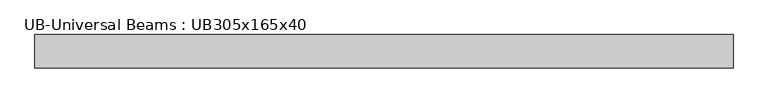
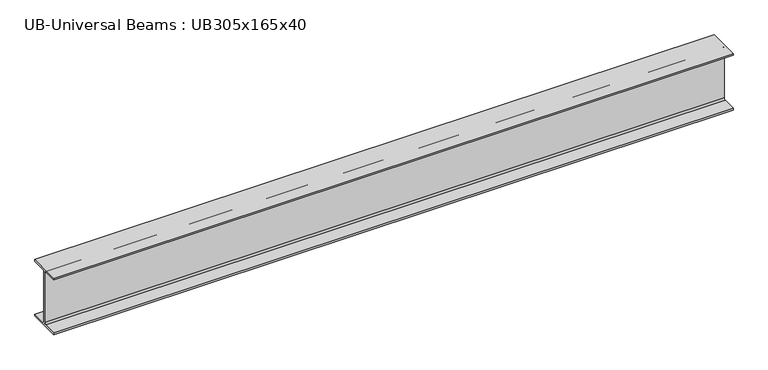
"""IFC4 building model written with IfcOpenShell, lengths in millimetres: beam geometry, UB-Universal Beams : UB305x165x40."""

from ifc_helpers import new_model, si_unit, point, frame, frame_2d, origin, place, context, project, spatial, polyline, circle_curve, trimmed, segment, composite_curve, outline, extrude, source, transform, mapped, element, save


def ub_universal_beams_ub305x165x40_daa15f39(model_context):
    return source(origin(), model_context, "Body", "SweptSolid", [
        extrude(outline(composite_curve([segment(polyline([(82.5, -141.5), (82.5, -151.7), (-82.5, -151.7), (-82.5, -141.5), (-11.9, -141.5)]), True, "CONTINUOUS"), segment(trimmed(circle_curve(frame_2d((-11.9, -132.6)), 8.9), [point((-11.9, -141.5))], [point((-3.0, -132.6))], True, "CARTESIAN"), True, "CONTINUOUS"), segment(polyline([(-3.0, -132.6), (-3.0, 132.6)]), True, "CONTINUOUS"), segment(trimmed(circle_curve(frame_2d((-11.9, 132.6)), 8.9), [point((-3.0, 132.6))], [point((-11.9, 141.5))], True, "CARTESIAN"), True, "CONTINUOUS"), segment(polyline([(-11.9, 141.5), (-82.5, 141.5), (-82.5, 151.7), (82.5, 151.7), (82.5, 141.5), (11.9, 141.5)]), True, "CONTINUOUS"), segment(trimmed(circle_curve(frame_2d((11.9, 132.6)), 8.9), [point((11.9, 141.5))], [point((3.0, 132.6))], True, "CARTESIAN"), True, "CONTINUOUS"), segment(polyline([(3.0, 132.6), (3.0, -132.6)]), True, "CONTINUOUS"), segment(trimmed(circle_curve(frame_2d((11.9, -132.6)), 8.9), [point((3.0, -132.6))], [point((11.9, -141.5))], True, "CARTESIAN"), True, "CONTINUOUS"), segment(polyline([(11.9, -141.5), (82.5, -141.5)]), True, "CONTINUOUS")], self_intersect=False)), frame((-1724.05, 0.0, 0.0), z_axis=(1.0, 0.0, 0.0), x_axis=(0.0, 1.0, 0.0)), (0.0, 0.0, 1.0), 3448.1),
    ])


if __name__ == "__main__":
    model = new_model("IFC4")
    model_context = context("Model", 3, world=origin())
    ifc_project = project(units=[si_unit("LENGTHUNIT", "METRE", prefix="MILLI")], contexts=[model_context])
    site = spatial("IfcSite", under=ifc_project)
    building = spatial("IfcBuilding", under=site)
    placement = place(None, origin())
    ub_universal_beams_ub305x165x40_shape = ub_universal_beams_ub305x165x40_daa15f39(model_context)
    element("IfcBeam", 1, ObjectType="UB-Universal Beams : UB305x165x40", at=placement, inside=building, context=model_context, shape_type="MappedRepresentation", body=[
        mapped(ub_universal_beams_ub305x165x40_shape, transform((0.0, 0.0, 0.0), x_axis=(1.0, 0.0, 0.0), y_axis=(0.0, 1.0, 0.0), z_axis=(0.0, 0.0, 1.0))),
    ])
    save(model, "model.ifc")

# Revit data of these elements
# Type "UB-Universal Beams : UB305x165x40"
#   Section Name Key = "UB305X165X40"
#   Width = 16.5 cm
#   Web Thickness = 0.6 cm
#   Web Fillet = 0.89 cm
#   Warping Constant = 164000.0 cm⁶
#   Torsional Moment of Inertia = 14.70 cm⁴
#   Section Area = 51.3 cm²
#   Plastic Modulus weak axis = 142.0 cm³
#   Plastic Modulus strong axis = 623.0 cm³
#   Nominal Weight = 40.2999 kgf/m
#   Moment of Inertia weak axis = 764.00 cm⁴
#   Moment of Inertia strong axis = 8503.00 cm⁴
#   Height = 30.34 cm
#   Flange Thickness = 1.02 cm
#   Elastic Modulus weak axis = 92.6 cm³
#   Elastic Modulus strong axis = 560.0 cm³
#   Centroid Vertical = 15.17 cm
#   Centroid Horizontal = 8.25 cm
#   Bolt Spacing = 9.0 cm
#   Length [instance default] = 1500 mm
#   Structural Material [instance default] = Metal - Steel 43-275
#   Type Comments = ""
#   Assembly Code = ""
# Element 1 (IfcBeam, "UB-Universal Beams : UB305x165x40")
#   Materials on its faces: "Metal - Steel 43-275"
# Materials
#   "Metal - Steel 43-275": class "Metal", colour RGB 247 247 247, transparency 0, Cost = 0
